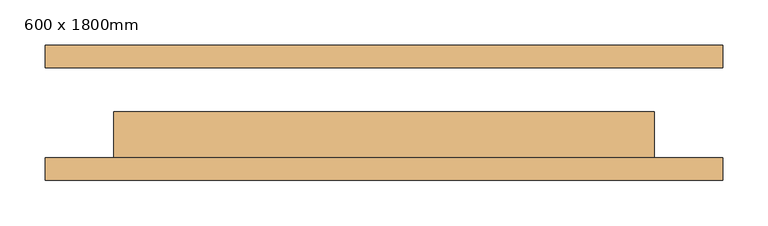
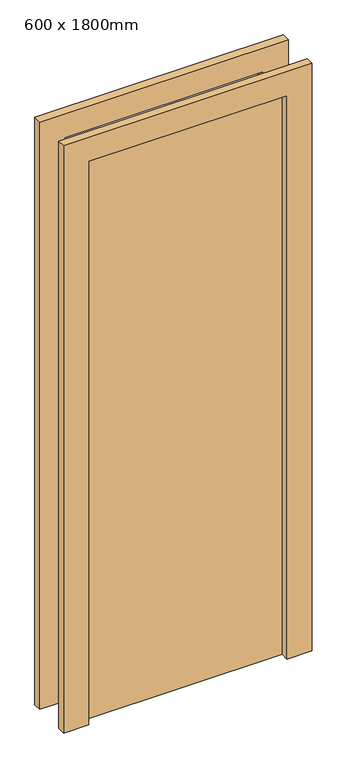
"""IFC4 building model written with IfcOpenShell, lengths in millimetres: door geometry, 单扇 - 与墙齐 : 600 x 1800mm."""

from ifc_helpers import new_model, si_unit, frame, origin, origin_with_axes, place, context, project, spatial, polyline, outline, extrude, source, transform, mapped, element, save


def door_600_x_1800mm_26a27b96(model_context):
    return source(origin(), model_context, "Body", "SweptSolid", [
        extrude(outline(polyline([(1876.0, -376.0), (0.0, -376.0), (0.0, -300.0), (1800.0, -300.0), (1800.0, 300.0), (0.0, 300.0), (0.0, 376.0), (1876.0, 376.0), (1876.0, -376.0)])), frame((0.0, -75.0, 0.0), z_axis=(0.0, 1.0, 0.0), x_axis=(0.0, 0.0, 1.0)), (0.0, 0.0, 1.0), 25.0),
        extrude(outline(polyline([(1876.0, 376.0), (1876.0, -376.0), (0.0, -376.0), (0.0, -300.0), (1800.0, -300.0), (1800.0, 300.0), (0.0, 300.0), (0.0, 376.0), (1876.0, 376.0)])), frame((0.0, 50.0, 0.0), z_axis=(0.0, 1.0, 0.0), x_axis=(0.0, 0.0, 1.0)), (0.0, 0.0, 1.0), 25.0),
        extrude(outline(polyline([(300.0, 1.0), (300.0, -50.0), (-300.0, -50.0), (-300.0, 1.0), (300.0, 1.0)])), origin_with_axes(), (0.0, 0.0, 1.0), 1800.0),
    ])


if __name__ == "__main__":
    model = new_model("IFC4")
    model_context = context("Model", 3, world=origin())
    ifc_project = project(units=[si_unit("LENGTHUNIT", "METRE", prefix="MILLI")], contexts=[model_context])
    site = spatial("IfcSite", under=ifc_project)
    building = spatial("IfcBuilding", under=site)
    placement = place(None, origin())
    door_600_x_1800mm_shape = door_600_x_1800mm_26a27b96(model_context)
    element("IfcDoor", 1, ObjectType="单扇 - 与墙齐 : 600 x 1800mm", at=placement, inside=building, context=model_context, shape_type="MappedRepresentation", body=[
        mapped(door_600_x_1800mm_shape, transform((0.0, 0.0, 0.0), x_axis=(1.0, 0.0, 0.0), y_axis=(0.0, 1.0, 0.0), z_axis=(0.0, 0.0, 1.0))),
    ])
    save(model, "model.ifc")

# Revit data of these elements
# Type "单扇 - 与墙齐 : 600 x 1800mm"
#   Type Mark = "M0618"
#   Construction Type Id = "MDOOR"
#   Analytic Construction = "金属"
#   贴面宽度 = 76 mm
#   贴面投影内部 = 25 mm
#   贴面投影外部 = 25 mm
#   Thickness = 51 mm
#   Height = 1800 mm
#   Width = 600 mm
#   Heat Transfer Coefficient (U) = 3.7021 W/(m²·K)
#   框架材质 = 门 - 框架
#   门材质 = 门 - 嵌板
#   Visual Light Transmittance = 0
#   Solar Heat Gain Coefficient = 0
#   Wall Closure = (empty or 0)
#   Function = (empty or 0)
# Element 1 (IfcDoor, "单扇 - 与墙齐 : 600 x 1800mm")
#   Materials on its faces: "门 - 框架", "门 - 嵌板"
# Materials
#   "门 - 框架": class "其他", colour RGB 118 70 51, transparency 0, Cost = 0
#   "门 - 嵌板": class "木质", colour RGB 210 159 95, transparency 0, Cost = 0
